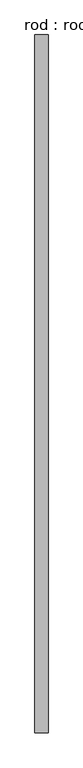
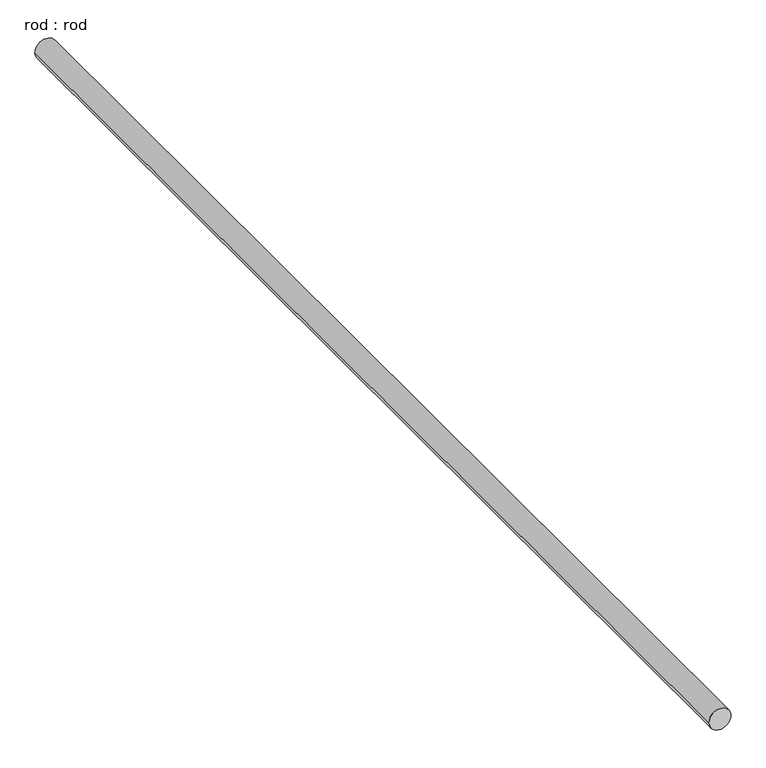
"""IFC4 building model written with IfcOpenShell, lengths in millimetres: proxy geometry, rod : rod."""

import ifcopenshell
import ifcopenshell.guid

model = None  # the IFC model being written
_history = None  # IfcOwnerHistory: only IFC2X3 demands one
_inside = {}  # id of a spatial element -> (the spatial element, [elements in it])
_under = {}  # id of a project, library or spatial element -> (it, [spatial elements below it])
_declared = {}  # id of a project -> (the project, [libraries it declares])
_typed = {}  # id of a type object -> (the type object, [elements of that type])
_made_of = {}  # id of a material, layer set ... -> (it, [elements and type objects made of it])


def new_model(schema):
    """Start an empty IFC model of exactly this schema.

    Asked for "IFC4X3", IfcOpenShell would pick the latest addendum, in which some entities
    have other attributes; the version numbers below select the first issue.
    IFC2X3 requires an IfcOwnerHistory on every rooted entity: one is made here for all.
    """
    global model, _history
    if schema == "IFC4X3":
        model = ifcopenshell.file(schema_version=(4, 3, 0, 0))
    else:
        model = ifcopenshell.file(schema=schema)
    _inside.clear()
    _under.clear()
    _declared.clear()
    _typed.clear()
    _made_of.clear()
    _history = None
    if model.schema == "IFC2X3":
        org = make("IfcOrganization", Name="unknown")
        user = make(
            "IfcPersonAndOrganization",
            ThePerson=make("IfcPerson", FamilyName="unknown"),
            TheOrganization=org,
        )
        app = make(
            "IfcApplication",
            ApplicationDeveloper=org,
            Version="unknown",
            ApplicationFullName="unknown",
            ApplicationIdentifier="unknown",
        )
        _history = make(
            "IfcOwnerHistory",
            OwningUser=user,
            OwningApplication=app,
            ChangeAction="ADDED",
            CreationDate=0,
        )
    return model


def make(cls, **values):
    """One entity of the class cls with the attributes given. An attribute that is None is left unset."""
    return model.create_entity(
        cls, **{name: value for name, value in values.items() if value is not None}
    )


def rooted(cls, **values):
    """An entity with a GlobalId (a new one), such as an element, a storey or a relation."""
    return make(cls, GlobalId=ifcopenshell.guid.new(), OwnerHistory=_history, **values)


def si_unit(unit_type, name, prefix=None):
    """IfcSIUnit, for example si_unit("LENGTHUNIT", "METRE", prefix="MILLI")."""
    return make("IfcSIUnit", UnitType=unit_type, Prefix=prefix, Name=name)


def assignment(units):
    """IfcUnitAssignment: the units of a project."""
    return None if units is None else make("IfcUnitAssignment", Units=units)


def point(xyz):
    """IfcCartesianPoint."""
    return None if xyz is None else make("IfcCartesianPoint", Coordinates=xyz)


def direction(xyz):
    """IfcDirection."""
    return None if xyz is None else make("IfcDirection", DirectionRatios=xyz)


def frame(location, z_axis=None, x_axis=None):
    """IfcAxis2Placement3D, a coordinate frame: its origin and axes. An axis left out is left unset."""
    return make(
        "IfcAxis2Placement3D",
        Location=point(location),
        Axis=direction(z_axis),
        RefDirection=direction(x_axis),
    )


def frame_2d(location, x_axis=None):
    """IfcAxis2Placement2D, a coordinate frame in the plane: its origin and x axis."""
    return make(
        "IfcAxis2Placement2D", Location=point(location), RefDirection=direction(x_axis)
    )


def origin():
    """The frame at (0, 0, 0) with its axes left unset."""
    return frame((0.0, 0.0, 0.0))


def place(relative_to, where):
    """IfcLocalPlacement: puts the frame where relative to a parent placement (None: the world)."""
    return make(
        "IfcLocalPlacement", PlacementRelTo=relative_to, RelativePlacement=where
    )


def context(
    kind, dimensions, precision=None, world=None, true_north=None, identifier=None
):
    """IfcGeometricRepresentationContext, for example the 3D "Model" context."""
    return make(
        "IfcGeometricRepresentationContext",
        ContextIdentifier=identifier,
        ContextType=kind,
        CoordinateSpaceDimension=dimensions,
        Precision=precision,
        WorldCoordinateSystem=world,
        TrueNorth=true_north,
    )


def project(units=None, contexts=None):
    """IfcProject with its units and contexts."""
    return rooted(
        "IfcProject",
        Name="project",
        RepresentationContexts=contexts,
        UnitsInContext=assignment(units),
    )


def spatial(cls, under=None, at=None, **own):
    """A site, building, storey or space (cls), placed at a placement, below another one or the project."""
    s = rooted(cls, ObjectPlacement=at, **own)
    if under is not None:
        _under.setdefault(under.id(), (under, []))[1].append(s)
    return s


def circle_curve(where, radius):
    """IfcCircle in the frame where."""
    return make("IfcCircle", Position=where, Radius=radius)


def trimmed(basis, trim1, trim2, sense, master):
    """IfcTrimmedCurve: the piece of a basis curve between two trims."""
    return make(
        "IfcTrimmedCurve",
        BasisCurve=basis,
        Trim1=trim1,
        Trim2=trim2,
        SenseAgreement=sense,
        MasterRepresentation=master,
    )


def segment(curve, same_sense, transition):
    """IfcCompositeCurveSegment."""
    return make(
        "IfcCompositeCurveSegment",
        Transition=transition,
        SameSense=same_sense,
        ParentCurve=curve,
    )


def composite_curve(segments, self_intersect=None):
    """IfcCompositeCurve: segments joined end to end."""
    return make("IfcCompositeCurve", Segments=segments, SelfIntersect=self_intersect)


def outline(outer, holes=None, kind="AREA"):
    """IfcArbitraryClosedProfileDef: a profile drawn as a closed curve; with holes, ...WithVoids."""
    if holes is None:
        return make("IfcArbitraryClosedProfileDef", ProfileType=kind, OuterCurve=outer)
    return make(
        "IfcArbitraryProfileDefWithVoids",
        ProfileType=kind,
        OuterCurve=outer,
        InnerCurves=holes,
    )


def extrude(swept, where, along, depth):
    """IfcExtrudedAreaSolid: the profile swept, set in the frame where, extruded along a direction by depth."""
    return make(
        "IfcExtrudedAreaSolid",
        SweptArea=swept,
        Position=where,
        ExtrudedDirection=direction(along),
        Depth=depth,
    )


def shape(context_of_items, identifier, shape_type, items):
    """IfcShapeRepresentation: the items that make up one representation, for example the "Body"."""
    return make(
        "IfcShapeRepresentation",
        ContextOfItems=context_of_items,
        RepresentationIdentifier=identifier,
        RepresentationType=shape_type,
        Items=items,
    )


def source(mapping_origin, context_of_items, identifier, shape_type, items):
    """IfcRepresentationMap: a shape defined once, which mapped items show again and again."""
    return make(
        "IfcRepresentationMap",
        MappingOrigin=mapping_origin,
        MappedRepresentation=shape(context_of_items, identifier, shape_type, items),
    )


def transform(
    local_origin,
    x_axis=None,
    y_axis=None,
    z_axis=None,
    scale=None,
    scale2=None,
    scale3=None,
    uniform=True,
):
    """IfcCartesianTransformationOperator3D, or its non-uniform kind. x_axis, y_axis, z_axis: its Axis1, 2, 3."""
    if uniform:
        return make(
            "IfcCartesianTransformationOperator3D",
            Axis1=direction(x_axis),
            Axis2=direction(y_axis),
            LocalOrigin=point(local_origin),
            Scale=scale,
            Axis3=direction(z_axis),
        )
    return make(
        "IfcCartesianTransformationOperator3DnonUniform",
        Axis1=direction(x_axis),
        Axis2=direction(y_axis),
        LocalOrigin=point(local_origin),
        Scale=scale,
        Axis3=direction(z_axis),
        Scale2=scale2,
        Scale3=scale3,
    )


def mapped(mapping_source, mapping_target):
    """IfcMappedItem: shows the shape of a source again, moved by a transform."""
    return make(
        "IfcMappedItem", MappingSource=mapping_source, MappingTarget=mapping_target
    )


def made_of(thing, what):
    """Note that an element or type object is made of a material, layer set ...; save() writes the relation."""
    if what is not None:
        _made_of.setdefault(what.id(), (what, []))[1].append(thing)
    return thing


def element(
    cls,
    number,
    at=None,
    inside=None,
    cuts=None,
    type_object=None,
    material=None,
    context=None,
    identifier="Body",
    shape_type=None,
    held_by="IfcProductDefinitionShape",
    body=None,
    shapes=None,
    **own,
):
    """One element of the class cls, such as IfcWall. Its Tag is "e" and its number.

    at: its placement. inside: the storey or other place that contains it. cuts: it is an
    opening in that element (IfcRelVoidsElement). A single representation is given by context,
    identifier, shape_type and body (its items); several are given by shapes. held_by: the class
    of the entity that holds the representations. save() writes the other relations.
    """
    e = rooted(cls, Tag="e%d" % number, ObjectPlacement=at, **own)
    if body is not None:
        shapes = [shape(context, identifier, shape_type, body)]
    if shapes is not None:
        e.Representation = make(held_by, Representations=shapes)
    if inside is not None:
        _inside.setdefault(inside.id(), (inside, []))[1].append(e)
    if cuts is not None:
        rooted(
            "IfcRelVoidsElement", RelatingBuildingElement=cuts, RelatedOpeningElement=e
        )
    if type_object is not None:
        _typed.setdefault(type_object.id(), (type_object, []))[1].append(e)
    return made_of(e, material)


def aggregate(whole, parts):
    """IfcRelAggregates: a whole, such as a stair, and the parts it consists of."""
    return rooted("IfcRelAggregates", RelatingObject=whole, RelatedObjects=parts)


def save(model, path):
    """Write the relations noted so far, then the file.

    IfcRelAggregates (storeys below a building ...), IfcRelContainedInSpatialStructure (elements
    in a storey), IfcRelDefinesByType, IfcRelAssociatesMaterial and IfcRelDeclares: one each for
    every whole, place, type object, material and project.
    """
    for whole, parts in _under.values():
        aggregate(whole, parts)
    for where, things in _inside.values():
        rooted(
            "IfcRelContainedInSpatialStructure",
            RelatedElements=things,
            RelatingStructure=where,
        )
    for kind, things in _typed.values():
        rooted("IfcRelDefinesByType", RelatedObjects=things, RelatingType=kind)
    for what, things in _made_of.values():
        rooted("IfcRelAssociatesMaterial", RelatedObjects=things, RelatingMaterial=what)
    for by, libraries in _declared.values():
        rooted("IfcRelDeclares", RelatingContext=by, RelatedDefinitions=libraries)
    model.write(path)


def rod_rod_51a05636(model_context):
    return source(origin(), model_context, "Body", "SweptSolid", [
        extrude(outline(composite_curve([segment(trimmed(circle_curve(frame_2d((0.0108462, 0.0)), 200.0), [point((0.0108462, 200.0))], [point((0.0108462, -200.0))], False, "CARTESIAN"), True, "CONTINUOUS"), segment(trimmed(circle_curve(frame_2d((0.0108462, 0.0)), 200.0), [point((0.0108462, -200.0))], [point((0.0108462, 200.0))], False, "CARTESIAN"), True, "CONTINUOUS")], self_intersect=False)), frame((0.0, -6502.1404259, 0.0), z_axis=(0.0, 1.0, 0.0), x_axis=(0.0, 0.0, 1.0)), (0.0, 0.0, 1.0), 21189.7380824),
    ])


if __name__ == "__main__":
    model = new_model("IFC4")
    model_context = context("Model", 3, world=origin())
    ifc_project = project(units=[si_unit("LENGTHUNIT", "METRE", prefix="MILLI")], contexts=[model_context])
    site = spatial("IfcSite", under=ifc_project)
    building = spatial("IfcBuilding", under=site)
    placement = place(None, origin())
    rod_rod_shape = rod_rod_51a05636(model_context)
    element("IfcBuildingElementProxy", 1, Name="rod : rod", ObjectType="rod : rod", at=placement, inside=building, context=model_context, shape_type="MappedRepresentation", body=[
        mapped(rod_rod_shape, transform((0.0, 0.0, 0.0), x_axis=(1.0, 0.0, 0.0), y_axis=(0.0, 1.0, 0.0), z_axis=(0.0, 0.0, 1.0))),
    ])
    save(model, "model.ifc")

# Revit data of these elements
# Type "rod : rod"
#   Default Elevation = 0
